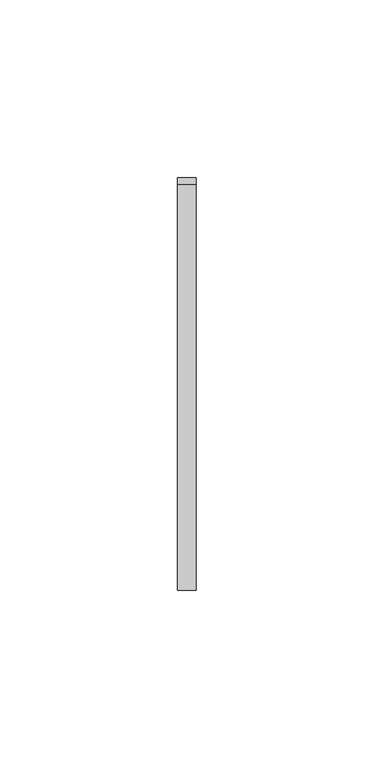
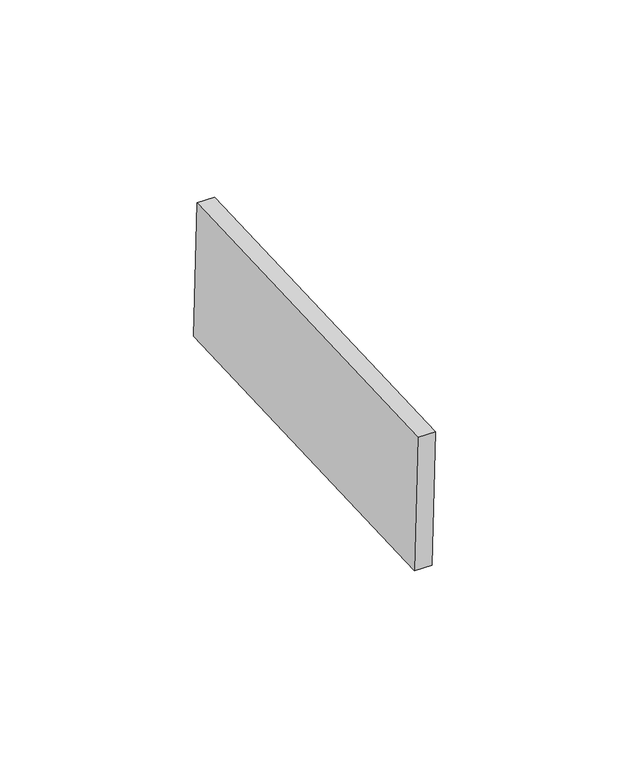
"""IFC4 building model written with IfcOpenShell, lengths in millimetres: proxy geometry, Inner panel:Inner panel:1:Inner panel:1 : Inner panel:Inner panel:300324:2:Inner panel:1:Inner panel:1 : Inner panel:Inner panel:300324:2 : Inner panel:Inner panel:1:Inner panel:1 : Inner panel:Inner panel:300324:300043:82 : Inner panel:Inner panel:1:Inner panel:1 : Inner panel:Inner panel:300324:2:Inner panel:1:Inner panel:1 : Inner panel:Inner panel:300324:2 : Inner panel:Inner panel:1:Inner panel:1 : Inner panel:Inner panel:300324:300043:308120."""

from ifc_helpers import new_model, si_unit, frame, origin, place, context, project, spatial, polyline, outline, extrude, source, transform, mapped, element, save


def generic_models_43b82a9b(model_context):
    return source(origin(), model_context, "Body", "SweptSolid", [
        extrude(outline(polyline([(0.0, -114.3), (0.0, 0.0), (5.2138089, 0.0), (5.2138089, -114.3), (0.0, -114.3)])), frame((592310.995117, -577458.3096573, 4016.6427799), z_axis=(0.0, -0.04163054471216399, 0.9991330730923527), x_axis=(-1.0, 0.0, 0.0)), (0.0, 0.0, 1.0), 43.2233908),
    ])


if __name__ == "__main__":
    model = new_model("IFC4")
    model_context = context("Model", 3, world=origin())
    ifc_project = project(units=[si_unit("LENGTHUNIT", "METRE", prefix="MILLI")], contexts=[model_context])
    site = spatial("IfcSite", under=ifc_project)
    building = spatial("IfcBuilding", under=site)
    placement = place(None, origin())
    generic_models_shape = generic_models_43b82a9b(model_context)
    element("IfcBuildingElementProxy", 1, Name="Inner panel:Inner panel:1:Inner panel:1 : Inner panel:Inner panel:300324:2:Inner panel:1:Inner panel:1 : Inner panel:Inner panel:300324:2 : Inner panel:Inner panel:1:Inner panel:1 : Inner panel:Inner panel:300324:300043:82 : Inner panel:Inner panel:1:Inner panel:1 : Inner panel:Inner panel:300324:2:Inner panel:1:Inner panel:1 : Inner panel:Inner panel:300324:2 : Inner panel:Inner panel:1:Inner panel:1 : Inner panel:Inner panel:300324:300043:308120", ObjectType="Inner panel:Inner panel:1:Inner panel:1 : Inner panel:Inner panel:300324:2:Inner panel:1:Inner panel:1 : Inner panel:Inner panel:300324:2 : Inner panel:Inner panel:1:Inner panel:1 : Inner panel:Inner panel:300324:300043:82 : Inner panel:Inner panel:1:Inner panel:1 : Inner panel:Inner panel:300324:2:Inner panel:1:Inner panel:1 : Inner panel:Inner panel:300324:2 : Inner panel:Inner panel:1:Inner panel:1 : Inner panel:Inner panel:300324:300043:308120", at=placement, inside=building, context=model_context, shape_type="MappedRepresentation", body=[
        mapped(generic_models_shape, transform((0.0, 0.0, 0.0), x_axis=(1.0, 0.0, 0.0), y_axis=(0.0, 1.0, 0.0), z_axis=(0.0, 0.0, 1.0))),
    ])
    save(model, "model.ifc")

# Revit data of these elements
# Type "Inner panel:Inner panel:1:Inner panel:1 : Inner panel:Inner panel:300324:2:Inner panel:1:Inner panel:1 : Inner panel:Inner panel:300324:2 : Inner panel:Inner panel:1:Inner panel:1 : Inner panel:Inner panel:300324:300043:82 : Inner panel:Inner panel:1:Inner panel:1 : Inner panel:Inner panel:300324:2:Inner panel:1:Inner panel:1 : Inner panel:Inner panel:300324:2 : Inner panel:Inner panel:1:Inner panel:1 : Inner panel:Inner panel:300324:300043:308120"
#   NameOverride = "Inner panel:Inner panel:1:Inner panel:1 : Inner panel:Inner panel:300324:2:Inner panel:1:Inner panel:1 : Inner panel:Inner panel:300324:2 : Inner panel:Inner panel:1:Inner panel:1 : Inner panel:Inner panel:300324:300043:308120"
#   ObjectTypeOverride = "Inner panel:1:Inner panel:1 : Inner panel:Inner panel:300324:2 : Inner panel:Inner panel:1:Inner panel:1 : Inner panel:Inner panel:300324:300043"
#   Reference = "Inner panel"
#   Tag = "308120"
# Element 1 (IfcBuildingElementProxy, "Inner panel:Inner panel:1:Inner panel:1 : Inner panel:Inner panel:300324:2:Inner panel:1:Inner panel:1 : Inner panel:Inner panel:300324:2 : Inner panel:Inner panel:1:Inner panel:1 : Inner panel:Inner panel:300324:300043:82 : Inner panel:Inner panel:1:Inner panel:1 : Inner panel:Inner panel:300324:2:Inner panel:1:Inner panel:1 : Inner panel:Inner panel:300324:2 : Inner panel:Inner panel:1:Inner panel:1 : Inner panel:Inner panel:300324:300043:308120")
#   Materials on its faces: "SLIDING CLIP"
# Materials
#   "SLIDING CLIP": class "Generic", colour RGB 120 120 120, transparency 0, Cost = 0
